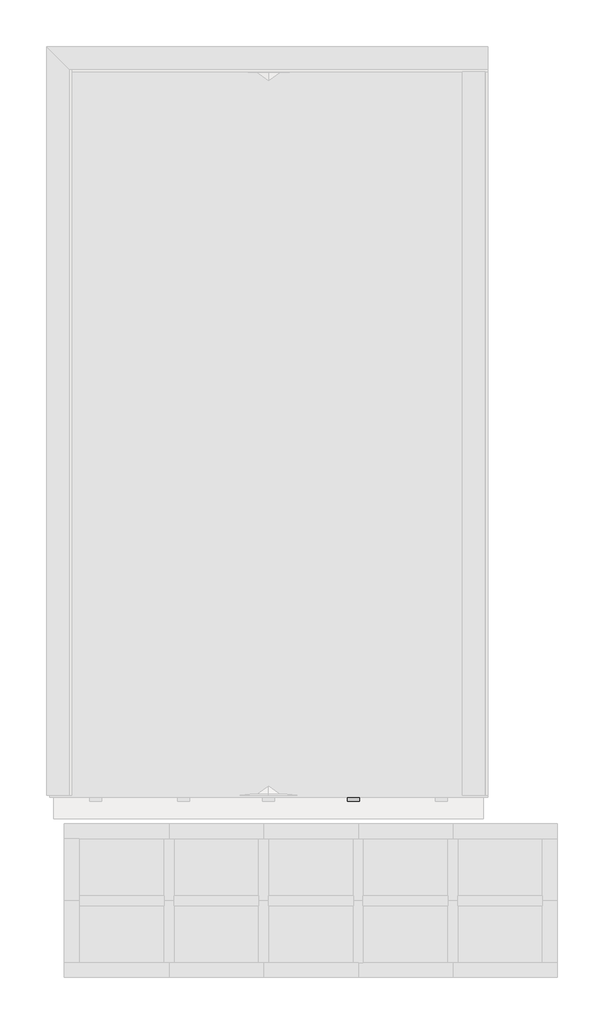
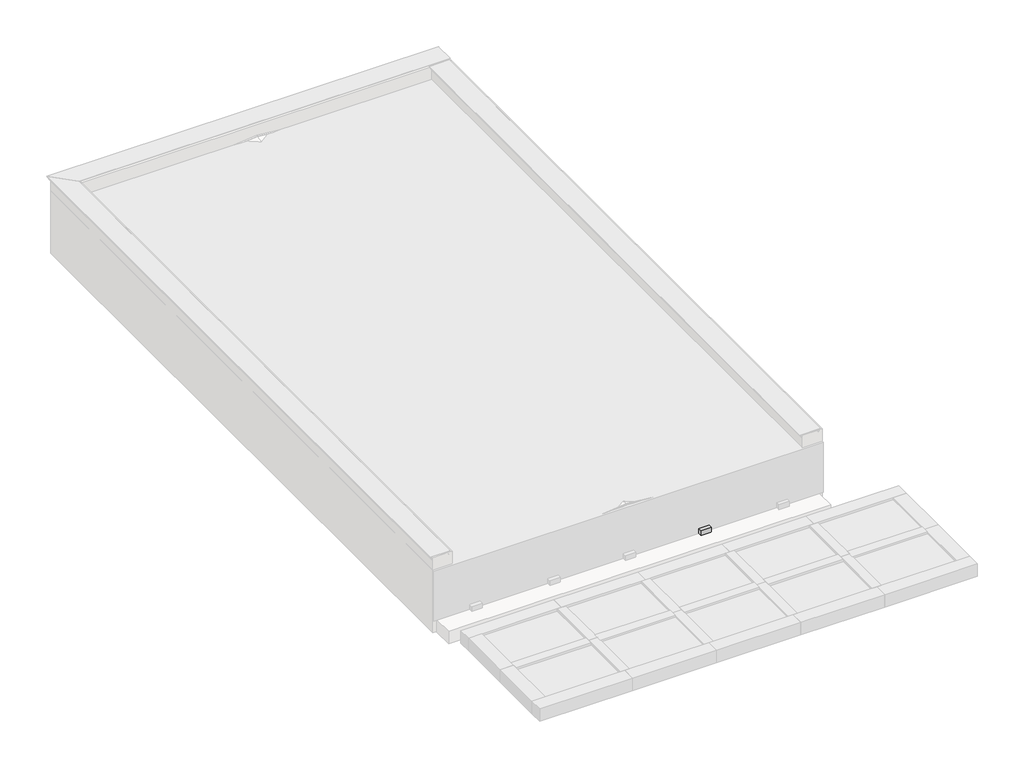
# One storey, part 2 of 3: 38 beams, 6 columns.
"""IFC4 building model written with IfcOpenShell, lengths in millimetres."""

import ifcopenshell
import ifcopenshell.guid

model = None  # the IFC model being written
_history = None  # IfcOwnerHistory: only IFC2X3 demands one
_inside = {}  # id of a spatial element -> (the spatial element, [elements in it])
_under = {}  # id of a project, library or spatial element -> (it, [spatial elements below it])
_declared = {}  # id of a project -> (the project, [libraries it declares])
_typed = {}  # id of a type object -> (the type object, [elements of that type])
_made_of = {}  # id of a material, layer set ... -> (it, [elements and type objects made of it])


def new_model(schema):
    """Start an empty IFC model of exactly this schema.

    Asked for "IFC4X3", IfcOpenShell would pick the latest addendum, in which some entities
    have other attributes; the version numbers below select the first issue.
    IFC2X3 requires an IfcOwnerHistory on every rooted entity: one is made here for all.
    """
    global model, _history
    if schema == "IFC4X3":
        model = ifcopenshell.file(schema_version=(4, 3, 0, 0))
    else:
        model = ifcopenshell.file(schema=schema)
    _inside.clear()
    _under.clear()
    _declared.clear()
    _typed.clear()
    _made_of.clear()
    _history = None
    if model.schema == "IFC2X3":
        org = make("IfcOrganization", Name="unknown")
        user = make(
            "IfcPersonAndOrganization",
            ThePerson=make("IfcPerson", FamilyName="unknown"),
            TheOrganization=org,
        )
        app = make(
            "IfcApplication",
            ApplicationDeveloper=org,
            Version="unknown",
            ApplicationFullName="unknown",
            ApplicationIdentifier="unknown",
        )
        _history = make(
            "IfcOwnerHistory",
            OwningUser=user,
            OwningApplication=app,
            ChangeAction="ADDED",
            CreationDate=0,
        )
    return model


def make(cls, **values):
    """One entity of the class cls with the attributes given. An attribute that is None is left unset."""
    return model.create_entity(
        cls, **{name: value for name, value in values.items() if value is not None}
    )


def rooted(cls, **values):
    """An entity with a GlobalId (a new one), such as an element, a storey or a relation."""
    return make(cls, GlobalId=ifcopenshell.guid.new(), OwnerHistory=_history, **values)


def si_unit(unit_type, name, prefix=None):
    """IfcSIUnit, for example si_unit("LENGTHUNIT", "METRE", prefix="MILLI")."""
    return make("IfcSIUnit", UnitType=unit_type, Prefix=prefix, Name=name)


def assignment(units):
    """IfcUnitAssignment: the units of a project."""
    return None if units is None else make("IfcUnitAssignment", Units=units)


def point(xyz):
    """IfcCartesianPoint."""
    return None if xyz is None else make("IfcCartesianPoint", Coordinates=xyz)


def direction(xyz):
    """IfcDirection."""
    return None if xyz is None else make("IfcDirection", DirectionRatios=xyz)


def frame(location, z_axis=None, x_axis=None):
    """IfcAxis2Placement3D, a coordinate frame: its origin and axes. An axis left out is left unset."""
    return make(
        "IfcAxis2Placement3D",
        Location=point(location),
        Axis=direction(z_axis),
        RefDirection=direction(x_axis),
    )


def frame_2d(location, x_axis=None):
    """IfcAxis2Placement2D, a coordinate frame in the plane: its origin and x axis."""
    return make(
        "IfcAxis2Placement2D", Location=point(location), RefDirection=direction(x_axis)
    )


def origin():
    """The frame at (0, 0, 0) with its axes left unset."""
    return frame((0.0, 0.0, 0.0))


def place(relative_to, where):
    """IfcLocalPlacement: puts the frame where relative to a parent placement (None: the world)."""
    return make(
        "IfcLocalPlacement", PlacementRelTo=relative_to, RelativePlacement=where
    )


def context(
    kind, dimensions, precision=None, world=None, true_north=None, identifier=None
):
    """IfcGeometricRepresentationContext, for example the 3D "Model" context."""
    return make(
        "IfcGeometricRepresentationContext",
        ContextIdentifier=identifier,
        ContextType=kind,
        CoordinateSpaceDimension=dimensions,
        Precision=precision,
        WorldCoordinateSystem=world,
        TrueNorth=true_north,
    )


def project(units=None, contexts=None):
    """IfcProject with its units and contexts."""
    return rooted(
        "IfcProject",
        Name="project",
        RepresentationContexts=contexts,
        UnitsInContext=assignment(units),
    )


def spatial(cls, under=None, at=None, **own):
    """A site, building, storey or space (cls), placed at a placement, below another one or the project."""
    s = rooted(cls, ObjectPlacement=at, **own)
    if under is not None:
        _under.setdefault(under.id(), (under, []))[1].append(s)
    return s


def polyline(points):
    """IfcPolyline through the points."""
    return make("IfcPolyline", Points=[point(p) for p in points])


def circle_curve(where, radius):
    """IfcCircle in the frame where."""
    return make("IfcCircle", Position=where, Radius=radius)


def trimmed(basis, trim1, trim2, sense, master):
    """IfcTrimmedCurve: the piece of a basis curve between two trims."""
    return make(
        "IfcTrimmedCurve",
        BasisCurve=basis,
        Trim1=trim1,
        Trim2=trim2,
        SenseAgreement=sense,
        MasterRepresentation=master,
    )


def segment(curve, same_sense, transition):
    """IfcCompositeCurveSegment."""
    return make(
        "IfcCompositeCurveSegment",
        Transition=transition,
        SameSense=same_sense,
        ParentCurve=curve,
    )


def composite_curve(segments, self_intersect=None):
    """IfcCompositeCurve: segments joined end to end."""
    return make("IfcCompositeCurve", Segments=segments, SelfIntersect=self_intersect)


def outline(outer, holes=None, kind="AREA"):
    """IfcArbitraryClosedProfileDef: a profile drawn as a closed curve; with holes, ...WithVoids."""
    if holes is None:
        return make("IfcArbitraryClosedProfileDef", ProfileType=kind, OuterCurve=outer)
    return make(
        "IfcArbitraryProfileDefWithVoids",
        ProfileType=kind,
        OuterCurve=outer,
        InnerCurves=holes,
    )


def extrude(swept, where, along, depth):
    """IfcExtrudedAreaSolid: the profile swept, set in the frame where, extruded along a direction by depth."""
    return make(
        "IfcExtrudedAreaSolid",
        SweptArea=swept,
        Position=where,
        ExtrudedDirection=direction(along),
        Depth=depth,
    )


def shape(context_of_items, identifier, shape_type, items):
    """IfcShapeRepresentation: the items that make up one representation, for example the "Body"."""
    return make(
        "IfcShapeRepresentation",
        ContextOfItems=context_of_items,
        RepresentationIdentifier=identifier,
        RepresentationType=shape_type,
        Items=items,
    )


def source(mapping_origin, context_of_items, identifier, shape_type, items):
    """IfcRepresentationMap: a shape defined once, which mapped items show again and again."""
    return make(
        "IfcRepresentationMap",
        MappingOrigin=mapping_origin,
        MappedRepresentation=shape(context_of_items, identifier, shape_type, items),
    )


def transform(
    local_origin,
    x_axis=None,
    y_axis=None,
    z_axis=None,
    scale=None,
    scale2=None,
    scale3=None,
    uniform=True,
):
    """IfcCartesianTransformationOperator3D, or its non-uniform kind. x_axis, y_axis, z_axis: its Axis1, 2, 3."""
    if uniform:
        return make(
            "IfcCartesianTransformationOperator3D",
            Axis1=direction(x_axis),
            Axis2=direction(y_axis),
            LocalOrigin=point(local_origin),
            Scale=scale,
            Axis3=direction(z_axis),
        )
    return make(
        "IfcCartesianTransformationOperator3DnonUniform",
        Axis1=direction(x_axis),
        Axis2=direction(y_axis),
        LocalOrigin=point(local_origin),
        Scale=scale,
        Axis3=direction(z_axis),
        Scale2=scale2,
        Scale3=scale3,
    )


def mapped(mapping_source, mapping_target):
    """IfcMappedItem: shows the shape of a source again, moved by a transform."""
    return make(
        "IfcMappedItem", MappingSource=mapping_source, MappingTarget=mapping_target
    )


def made_of(thing, what):
    """Note that an element or type object is made of a material, layer set ...; save() writes the relation."""
    if what is not None:
        _made_of.setdefault(what.id(), (what, []))[1].append(thing)
    return thing


def element(
    cls,
    number,
    at=None,
    inside=None,
    cuts=None,
    type_object=None,
    material=None,
    context=None,
    identifier="Body",
    shape_type=None,
    held_by="IfcProductDefinitionShape",
    body=None,
    shapes=None,
    **own,
):
    """One element of the class cls, such as IfcWall. Its Tag is "e" and its number.

    at: its placement. inside: the storey or other place that contains it. cuts: it is an
    opening in that element (IfcRelVoidsElement). A single representation is given by context,
    identifier, shape_type and body (its items); several are given by shapes. held_by: the class
    of the entity that holds the representations. save() writes the other relations.
    """
    e = rooted(cls, Tag="e%d" % number, ObjectPlacement=at, **own)
    if body is not None:
        shapes = [shape(context, identifier, shape_type, body)]
    if shapes is not None:
        e.Representation = make(held_by, Representations=shapes)
    if inside is not None:
        _inside.setdefault(inside.id(), (inside, []))[1].append(e)
    if cuts is not None:
        rooted(
            "IfcRelVoidsElement", RelatingBuildingElement=cuts, RelatedOpeningElement=e
        )
    if type_object is not None:
        _typed.setdefault(type_object.id(), (type_object, []))[1].append(e)
    return made_of(e, material)


def aggregate(whole, parts):
    """IfcRelAggregates: a whole, such as a stair, and the parts it consists of."""
    return rooted("IfcRelAggregates", RelatingObject=whole, RelatedObjects=parts)


def save(model, path):
    """Write the relations noted so far, then the file.

    IfcRelAggregates (storeys below a building ...), IfcRelContainedInSpatialStructure (elements
    in a storey), IfcRelDefinesByType, IfcRelAssociatesMaterial and IfcRelDeclares: one each for
    every whole, place, type object, material and project.
    """
    for whole, parts in _under.values():
        aggregate(whole, parts)
    for where, things in _inside.values():
        rooted(
            "IfcRelContainedInSpatialStructure",
            RelatedElements=things,
            RelatingStructure=where,
        )
    for kind, things in _typed.values():
        rooted("IfcRelDefinesByType", RelatedObjects=things, RelatingType=kind)
    for what, things in _made_of.values():
        rooted("IfcRelAssociatesMaterial", RelatedObjects=things, RelatingMaterial=what)
    for by, libraries in _declared.values():
        rooted("IfcRelDeclares", RelatingContext=by, RelatedDefinitions=libraries)
    model.write(path)


def cumeeira_telha_ondulada_fibrocimento_28917381(model_context):
    return source(origin(), model_context, "Body", "SweptSolid", [
        extrude(outline(composite_curve([segment(polyline([(58.3970135, 42.4437972), (53.9055884, 40.2467307)]), True, "CONTINUOUS"), segment(trimmed(circle_curve(frame_2d((-1.6029865, 13.0936483)), 61.7939461), [point((53.9055884, 40.2467307))], [point((-57.1115615, 40.2467307))], True, "CARTESIAN"), True, "CONTINUOUS"), segment(polyline([(-57.1115615, 40.2467307), (-61.6029865, 42.4437972)]), True, "CONTINUOUS"), segment(trimmed(circle_curve(frame_2d((-1.6029865, 13.0936483)), 66.7939461), [point((-61.6029865, 42.4437972))], [point((58.3970135, 42.4437972))], False, "CARTESIAN"), True, "CONTINUOUS")], self_intersect=False)), frame((-3626.5, 0.0, 0.0), z_axis=(1.0, 0.0, 0.0), x_axis=(0.0, 1.0, 0.0)), (0.0, 0.0, 1.0), 7253.0),
    ])


def viga_cumeeira_6x16cm_d80f05ee(model_context):
    return source(origin(), model_context, "Body", "SweptSolid", [
        extrude(outline(polyline([(3626.5, 30.0), (3626.5, -30.0), (-3626.5, -30.0), (-3626.5, 30.0), (3626.5, 30.0)])), frame((0.0, 0.0, -80.0), z_axis=(0.0, 0.0, 1.0), x_axis=(1.0, 0.0, 0.0)), (0.0, 0.0, 1.0), 160.0),
    ])


def column_1cffec27(model_context):
    return source(origin(), model_context, "Body", "SweptSolid", [
        extrude(outline(polyline([(30.0, 80.0), (30.0, -80.0), (-30.0, -80.0), (-30.0, 80.0), (30.0, 80.0)])), frame((0.0, 0.0, 3110.0), z_axis=(0.0, 0.0, 1.0), x_axis=(1.0, 0.0, 0.0)), (0.0, 0.0, 1.0), 238.0),
    ])


def column_35730ad5(model_context):
    return source(origin(), model_context, "Body", "SweptSolid", [
        extrude(outline(polyline([(30.0, 80.0), (30.0, -80.0), (-30.0, -80.0), (-30.0, 80.0), (30.0, 80.0)])), frame((0.0, 0.0, 3110.0), z_axis=(0.0, 0.0, 1.0), x_axis=(1.0, 0.0, 0.0)), (0.0, 0.0, 1.0), 197.9),
    ])


def column_00c463e4(model_context):
    return source(origin(), model_context, "Body", "SweptSolid", [
        extrude(outline(polyline([(30.0, 80.0), (30.0, -80.0), (-30.0, -80.0), (-30.0, 80.0), (30.0, 80.0)])), frame((0.0, 0.0, 3110.0), z_axis=(0.0, 0.0, 1.0), x_axis=(1.0, 0.0, 0.0)), (0.0, 0.0, 1.0), 109.8),
    ])


model = new_model("IFC4")

# Units and contexts
model_context = context("Model", 3, world=origin())
ifc_project = project(units=[si_unit("LENGTHUNIT", "METRE", prefix="MILLI")], contexts=[model_context])

# Site, building, storey
site = spatial("IfcSite", under=ifc_project)
building = spatial("IfcBuilding", under=site)
storey = spatial("IfcBuildingStorey", under=building, Name="COB. GARAGEM", Elevation=3050.0)

# Beams
placement = place(None, origin())
element("IfcBeam", 1, ObjectType="Madeira de lei : Berço 6x12cm", at=placement, inside=storey, context=model_context, shape_type="SweptSolid", body=[
    extrude(outline(polyline([(-9620.281307, 4423.9300153), (-9500.281307, 4423.9300153), (-9500.281307, 2423.9300153), (-9620.281307, 2423.9300153), (-9620.281307, 4423.9300153)])), frame((0.0, 0.0, 3050.0), z_axis=(0.0, 0.0, 1.0), x_axis=(1.0, 0.0, 0.0)), (0.0, 0.0, 1.0), 60.0),
])
element("IfcBeam", 2, ObjectType="Madeira de lei : Berço 6x12cm", at=placement, inside=storey, context=model_context, shape_type="SweptSolid", body=[
    extrude(outline(polyline([(-9620.281307, 2423.9300153), (-9500.281307, 2423.9300153), (-9500.281307, 423.9300153), (-9620.281307, 423.9300153), (-9620.281307, 2423.9300153)])), frame((0.0, 0.0, 3050.0), z_axis=(0.0, 0.0, 1.0), x_axis=(1.0, 0.0, 0.0)), (0.0, 0.0, 1.0), 60.0),
])
element("IfcBeam", 3, ObjectType="Madeira de lei : Berço 6x12cm", at=placement, inside=storey, context=model_context, shape_type="SweptSolid", body=[
    extrude(outline(polyline([(-8767.0824227, 4423.9300153), (-8647.0824227, 4423.9300153), (-8647.0824227, 2423.9300153), (-8767.0824227, 2423.9300153), (-8767.0824227, 4423.9300153)])), frame((0.0, 0.0, 3050.0), z_axis=(0.0, 0.0, 1.0), x_axis=(1.0, 0.0, 0.0)), (0.0, 0.0, 1.0), 60.0),
])
element("IfcBeam", 4, ObjectType="Madeira de lei : Berço 6x12cm", at=placement, inside=storey, context=model_context, shape_type="SweptSolid", body=[
    extrude(outline(polyline([(-8767.0824227, 2423.9300153), (-8647.0824227, 2423.9300153), (-8647.0824227, 423.9300153), (-8767.0824227, 423.9300153), (-8767.0824227, 2423.9300153)])), frame((0.0, 0.0, 3050.0), z_axis=(0.0, 0.0, 1.0), x_axis=(1.0, 0.0, 0.0)), (0.0, 0.0, 1.0), 60.0),
])
element("IfcBeam", 5, ObjectType="Madeira de lei : Berço 6x12cm", at=placement, inside=storey, context=model_context, shape_type="SweptSolid", body=[
    extrude(outline(polyline([(-8767.0824227, 423.9300153), (-8647.0824227, 423.9300153), (-8647.0824227, -236.0699847), (-8767.0824227, -236.0699847), (-8767.0824227, 423.9300153)])), frame((0.0, 0.0, 3050.0), z_axis=(0.0, 0.0, 1.0), x_axis=(1.0, 0.0, 0.0)), (0.0, 0.0, 1.0), 60.0),
])
element("IfcBeam", 6, ObjectType="Madeira de lei : Berço 6x12cm", at=placement, inside=storey, context=model_context, shape_type="SweptSolid", body=[
    extrude(outline(polyline([(-10473.4801913, 4423.9300153), (-10353.4801913, 4423.9300153), (-10353.4801913, 2423.9300153), (-10473.4801913, 2423.9300153), (-10473.4801913, 4423.9300153)])), frame((0.0, 0.0, 3050.0), z_axis=(0.0, 0.0, 1.0), x_axis=(1.0, 0.0, 0.0)), (0.0, 0.0, 1.0), 60.0),
])
element("IfcBeam", 7, ObjectType="Madeira de lei : Berço 6x12cm", at=placement, inside=storey, context=model_context, shape_type="SweptSolid", body=[
    extrude(outline(polyline([(-11356.5301913, 4423.9300153), (-11236.5301913, 4423.9300153), (-11236.5301913, 2423.9300153), (-11356.5301913, 2423.9300153), (-11356.5301913, 4423.9300153)])), frame((0.0, 0.0, 3050.0), z_axis=(0.0, 0.0, 1.0), x_axis=(1.0, 0.0, 0.0)), (0.0, 0.0, 1.0), 60.0),
])
cumeeira_telha_ondulada_fibrocimento_shape = cumeeira_telha_ondulada_fibrocimento_28917381(model_context)
element("IfcBeam", 8, ObjectType="Cumeeira Telha Ondulada : Fibrocimento", at=placement, inside=storey, context=model_context, shape_type="MappedRepresentation", body=[
    mapped(cumeeira_telha_ondulada_fibrocimento_shape, transform((-9560.281307, 3455.9300153, 3545.9751229), x_axis=(0.0, -1.0, 0.0), y_axis=(1.0, 0.0, 0.0), z_axis=(0.0, 0.0, 1.0))),
])
element("IfcBeam", 9, ObjectType="Telha Ondulada : Fibrocimento", at=placement, inside=storey, context=model_context, shape_type="SweptSolid", body=[
    extrude(outline(composite_curve([segment(trimmed(circle_curve(frame_2d((-58.7002979, -53.2060538)), 66.7939461), [point((-29.350149, 6.7939462))], [point((-29.350149, -113.2060538))], False, "CARTESIAN"), True, "CONTINUOUS"), segment(polyline([(-29.350149, -113.2060538), (-31.5472155, -108.7146288)]), True, "CONTINUOUS"), segment(trimmed(circle_curve(frame_2d((-58.7002979, -53.2060538)), 61.7939461), [point((-31.5472155, -108.7146288))], [point((-31.5472155, 2.3025211))], True, "CARTESIAN"), True, "CONTINUOUS"), segment(trimmed(circle_curve(frame_2d((0.0, 66.7939462)), 71.7939461), [point((-31.5472155, 2.3025211))], [point((-31.5472155, 131.2853712))], False, "CARTESIAN"), True, "CONTINUOUS"), segment(polyline([(-31.5472155, 131.2853712), (-29.350149, 126.7939462)]), True, "CONTINUOUS"), segment(trimmed(circle_curve(frame_2d((0.0, 66.7939462)), 66.7939461), [point((-29.350149, 126.7939462))], [point((-29.350149, 6.7939462))], True, "CARTESIAN"), True, "CONTINUOUS")], self_intersect=False)), frame((-11446.918865, 2229.326948, 3394.3067746), z_axis=(0.9950371902099892, 0.0, 0.09950371902099919), x_axis=(-0.09950371902099919, 0.0, 0.9950371902099892)), (0.0, 0.0, 1.0), 1886.8678854),
])
element("IfcBeam", 10, ObjectType="Telha Ondulada : Fibrocimento", at=placement, inside=storey, context=model_context, shape_type="SweptSolid", body=[
    extrude(outline(composite_curve([segment(trimmed(circle_curve(frame_2d((-58.7002979, -53.2060538)), 66.7939461), [point((-29.350149, 6.7939462))], [point((-29.350149, -113.2060538))], False, "CARTESIAN"), True, "CONTINUOUS"), segment(polyline([(-29.350149, -113.2060538), (-31.5472155, -108.7146288)]), True, "CONTINUOUS"), segment(trimmed(circle_curve(frame_2d((-58.7002979, -53.2060538)), 61.7939461), [point((-31.5472155, -108.7146288))], [point((-31.5472155, 2.3025211))], True, "CARTESIAN"), True, "CONTINUOUS"), segment(trimmed(circle_curve(frame_2d((0.0, 66.7939462)), 71.7939461), [point((-31.5472155, 2.3025211))], [point((-31.5472155, 131.2853712))], False, "CARTESIAN"), True, "CONTINUOUS"), segment(polyline([(-31.5472155, 131.2853712), (-29.350149, 126.7939462)]), True, "CONTINUOUS"), segment(trimmed(circle_curve(frame_2d((0.0, 66.7939462)), 66.7939461), [point((-29.350149, 126.7939462))], [point((-29.350149, 6.7939462))], True, "CARTESIAN"), True, "CONTINUOUS")], self_intersect=False)), frame((-11446.918865, 2473.826948, 3394.3067746), z_axis=(0.9950371902099892, 0.0, 0.09950371902099932), x_axis=(-0.09950371902099932, 0.0, 0.9950371902099892)), (0.0, 0.0, 1.0), 1886.8678854),
])
element("IfcBeam", 11, ObjectType="Telha Ondulada : Fibrocimento", at=placement, inside=storey, context=model_context, shape_type="SweptSolid", body=[
    extrude(outline(composite_curve([segment(trimmed(circle_curve(frame_2d((-58.7002979, -53.2060538)), 66.7939461), [point((-29.350149, 6.7939462))], [point((-29.350149, -113.2060538))], False, "CARTESIAN"), True, "CONTINUOUS"), segment(polyline([(-29.350149, -113.2060538), (-31.5472155, -108.7146288)]), True, "CONTINUOUS"), segment(trimmed(circle_curve(frame_2d((-58.7002979, -53.2060538)), 61.7939461), [point((-31.5472155, -108.7146288))], [point((-31.5472155, 2.3025211))], True, "CARTESIAN"), True, "CONTINUOUS"), segment(trimmed(circle_curve(frame_2d((0.0, 66.7939462)), 71.7939461), [point((-31.5472155, 2.3025211))], [point((-31.5472155, 131.2853712))], False, "CARTESIAN"), True, "CONTINUOUS"), segment(polyline([(-31.5472155, 131.2853712), (-29.350149, 126.7939462)]), True, "CONTINUOUS"), segment(trimmed(circle_curve(frame_2d((0.0, 66.7939462)), 66.7939461), [point((-29.350149, 126.7939462))], [point((-29.350149, 6.7939462))], True, "CARTESIAN"), True, "CONTINUOUS")], self_intersect=False)), frame((-11446.918865, 2718.326948, 3394.3067746), z_axis=(0.9950371902099892, 0.0, 0.09950371902099937), x_axis=(-0.09950371902099937, 0.0, 0.9950371902099892)), (0.0, 0.0, 1.0), 1886.8678854),
])
element("IfcBeam", 12, ObjectType="Telha Ondulada : Fibrocimento", at=placement, inside=storey, context=model_context, shape_type="SweptSolid", body=[
    extrude(outline(composite_curve([segment(trimmed(circle_curve(frame_2d((-58.7002979, -53.2060538)), 66.7939461), [point((-29.350149, 6.7939462))], [point((-29.350149, -113.2060538))], False, "CARTESIAN"), True, "CONTINUOUS"), segment(polyline([(-29.350149, -113.2060538), (-31.5472155, -108.7146288)]), True, "CONTINUOUS"), segment(trimmed(circle_curve(frame_2d((-58.7002979, -53.2060538)), 61.7939461), [point((-31.5472155, -108.7146288))], [point((-31.5472155, 2.3025211))], True, "CARTESIAN"), True, "CONTINUOUS"), segment(trimmed(circle_curve(frame_2d((0.0, 66.7939462)), 71.7939461), [point((-31.5472155, 2.3025211))], [point((-31.5472155, 131.2853712))], False, "CARTESIAN"), True, "CONTINUOUS"), segment(polyline([(-31.5472155, 131.2853712), (-29.350149, 126.7939462)]), True, "CONTINUOUS"), segment(trimmed(circle_curve(frame_2d((0.0, 66.7939462)), 66.7939461), [point((-29.350149, 126.7939462))], [point((-29.350149, 6.7939462))], True, "CARTESIAN"), True, "CONTINUOUS")], self_intersect=False)), frame((-11446.918865, 2962.826948, 3394.3067746), z_axis=(0.9950371902099892, 0.0, 0.09950371902099943), x_axis=(-0.09950371902099943, 0.0, 0.9950371902099892)), (0.0, 0.0, 1.0), 1886.8678854),
])
element("IfcBeam", 13, ObjectType="Telha Ondulada : Fibrocimento", at=placement, inside=storey, context=model_context, shape_type="SweptSolid", body=[
    extrude(outline(composite_curve([segment(trimmed(circle_curve(frame_2d((-58.7002979, -53.2060538)), 66.7939461), [point((-29.350149, 6.7939462))], [point((-29.350149, -113.2060538))], False, "CARTESIAN"), True, "CONTINUOUS"), segment(polyline([(-29.350149, -113.2060538), (-31.5472155, -108.7146288)]), True, "CONTINUOUS"), segment(trimmed(circle_curve(frame_2d((-58.7002979, -53.2060538)), 61.7939461), [point((-31.5472155, -108.7146288))], [point((-31.5472155, 2.3025211))], True, "CARTESIAN"), True, "CONTINUOUS"), segment(trimmed(circle_curve(frame_2d((0.0, 66.7939462)), 71.7939461), [point((-31.5472155, 2.3025211))], [point((-31.5472155, 131.2853712))], False, "CARTESIAN"), True, "CONTINUOUS"), segment(polyline([(-31.5472155, 131.2853712), (-29.350149, 126.7939462)]), True, "CONTINUOUS"), segment(trimmed(circle_curve(frame_2d((0.0, 66.7939462)), 66.7939461), [point((-29.350149, 126.7939462))], [point((-29.350149, 6.7939462))], True, "CARTESIAN"), True, "CONTINUOUS")], self_intersect=False)), frame((-11446.918865, 3207.326948, 3394.3067746), z_axis=(0.9950371902099892, 0.0, 0.09950371902099954), x_axis=(-0.09950371902099954, 0.0, 0.9950371902099892)), (0.0, 0.0, 1.0), 1886.8678854),
])
element("IfcBeam", 14, ObjectType="Telha Ondulada : Fibrocimento", at=placement, inside=storey, context=model_context, shape_type="SweptSolid", body=[
    extrude(outline(composite_curve([segment(trimmed(circle_curve(frame_2d((-58.7002979, -53.2060538)), 66.7939461), [point((-29.350149, 6.7939462))], [point((-29.350149, -113.2060538))], False, "CARTESIAN"), True, "CONTINUOUS"), segment(polyline([(-29.350149, -113.2060538), (-31.5472155, -108.7146288)]), True, "CONTINUOUS"), segment(trimmed(circle_curve(frame_2d((-58.7002979, -53.2060538)), 61.7939461), [point((-31.5472155, -108.7146288))], [point((-31.5472155, 2.3025211))], True, "CARTESIAN"), True, "CONTINUOUS"), segment(trimmed(circle_curve(frame_2d((0.0, 66.7939462)), 71.7939461), [point((-31.5472155, 2.3025211))], [point((-31.5472155, 131.2853712))], False, "CARTESIAN"), True, "CONTINUOUS"), segment(polyline([(-31.5472155, 131.2853712), (-29.350149, 126.7939462)]), True, "CONTINUOUS"), segment(trimmed(circle_curve(frame_2d((0.0, 66.7939462)), 66.7939461), [point((-29.350149, 126.7939462))], [point((-29.350149, 6.7939462))], True, "CARTESIAN"), True, "CONTINUOUS")], self_intersect=False)), frame((-11446.918865, 3451.826948, 3394.3067746), z_axis=(0.9950371902099892, 0.0, 0.09950371902099937), x_axis=(-0.09950371902099937, 0.0, 0.9950371902099892)), (0.0, 0.0, 1.0), 1886.8678854),
])
element("IfcBeam", 15, ObjectType="Telha Ondulada : Fibrocimento", at=placement, inside=storey, context=model_context, shape_type="SweptSolid", body=[
    extrude(outline(composite_curve([segment(trimmed(circle_curve(frame_2d((-58.7002979, -53.2060538)), 66.7939461), [point((-29.350149, 6.7939462))], [point((-29.350149, -113.2060538))], False, "CARTESIAN"), True, "CONTINUOUS"), segment(polyline([(-29.350149, -113.2060538), (-31.5472155, -108.7146288)]), True, "CONTINUOUS"), segment(trimmed(circle_curve(frame_2d((-58.7002979, -53.2060538)), 61.7939461), [point((-31.5472155, -108.7146288))], [point((-31.5472155, 2.3025211))], True, "CARTESIAN"), True, "CONTINUOUS"), segment(trimmed(circle_curve(frame_2d((0.0, 66.7939462)), 71.7939461), [point((-31.5472155, 2.3025211))], [point((-31.5472155, 131.2853712))], False, "CARTESIAN"), True, "CONTINUOUS"), segment(polyline([(-31.5472155, 131.2853712), (-29.350149, 126.7939462)]), True, "CONTINUOUS"), segment(trimmed(circle_curve(frame_2d((0.0, 66.7939462)), 66.7939461), [point((-29.350149, 126.7939462))], [point((-29.350149, 6.7939462))], True, "CARTESIAN"), True, "CONTINUOUS")], self_intersect=False)), frame((-11446.918865, 3696.326948, 3394.3067746), z_axis=(0.9950371902099892, 0.0, 0.09950371902099914), x_axis=(-0.09950371902099914, 0.0, 0.9950371902099892)), (0.0, 0.0, 1.0), 1886.8678854),
])
element("IfcBeam", 16, ObjectType="Telha Ondulada : Fibrocimento", at=placement, inside=storey, context=model_context, shape_type="SweptSolid", body=[
    extrude(outline(composite_curve([segment(trimmed(circle_curve(frame_2d((-58.7002979, -53.2060538)), 66.7939461), [point((-29.350149, 6.7939462))], [point((-29.350149, -113.2060538))], False, "CARTESIAN"), True, "CONTINUOUS"), segment(polyline([(-29.350149, -113.2060538), (-31.5472155, -108.7146288)]), True, "CONTINUOUS"), segment(trimmed(circle_curve(frame_2d((-58.7002979, -53.2060538)), 61.7939461), [point((-31.5472155, -108.7146288))], [point((-31.5472155, 2.3025211))], True, "CARTESIAN"), True, "CONTINUOUS"), segment(trimmed(circle_curve(frame_2d((0.0, 66.7939462)), 71.7939461), [point((-31.5472155, 2.3025211))], [point((-31.5472155, 131.2853712))], False, "CARTESIAN"), True, "CONTINUOUS"), segment(polyline([(-31.5472155, 131.2853712), (-29.350149, 126.7939462)]), True, "CONTINUOUS"), segment(trimmed(circle_curve(frame_2d((0.0, 66.7939462)), 66.7939461), [point((-29.350149, 126.7939462))], [point((-29.350149, 6.7939462))], True, "CARTESIAN"), True, "CONTINUOUS")], self_intersect=False)), frame((-11446.918865, 3940.826948, 3394.3067746), z_axis=(0.9950371902099892, 0.0, 0.09950371902099948), x_axis=(-0.09950371902099948, 0.0, 0.9950371902099892)), (0.0, 0.0, 1.0), 1886.8678854),
])
element("IfcBeam", 17, ObjectType="Telha Ondulada : Fibrocimento", at=placement, inside=storey, context=model_context, shape_type="SweptSolid", body=[
    extrude(outline(composite_curve([segment(trimmed(circle_curve(frame_2d((-58.7002979, -53.2060538)), 66.7939461), [point((-29.350149, 6.7939462))], [point((-29.350149, -113.2060538))], False, "CARTESIAN"), True, "CONTINUOUS"), segment(polyline([(-29.350149, -113.2060538), (-31.5472155, -108.7146288)]), True, "CONTINUOUS"), segment(trimmed(circle_curve(frame_2d((-58.7002979, -53.2060538)), 61.7939461), [point((-31.5472155, -108.7146288))], [point((-31.5472155, 2.3025211))], True, "CARTESIAN"), True, "CONTINUOUS"), segment(trimmed(circle_curve(frame_2d((0.0, 66.7939462)), 71.7939461), [point((-31.5472155, 2.3025211))], [point((-31.5472155, 131.2853712))], False, "CARTESIAN"), True, "CONTINUOUS"), segment(polyline([(-31.5472155, 131.2853712), (-29.350149, 126.7939462)]), True, "CONTINUOUS"), segment(trimmed(circle_curve(frame_2d((0.0, 66.7939462)), 66.7939461), [point((-29.350149, 126.7939462))], [point((-29.350149, 6.7939462))], True, "CARTESIAN"), True, "CONTINUOUS")], self_intersect=False)), frame((-11446.918865, 4185.326948, 3394.3067746), z_axis=(0.9950371902099892, 0.0, 0.09950371902099932), x_axis=(-0.09950371902099932, 0.0, 0.9950371902099892)), (0.0, 0.0, 1.0), 1886.8678854),
])
element("IfcBeam", 18, ObjectType="Telha Ondulada : Fibrocimento", at=placement, inside=storey, context=model_context, shape_type="SweptSolid", body=[
    extrude(outline(composite_curve([segment(trimmed(circle_curve(frame_2d((-58.7002979, -53.2060538)), 66.7939461), [point((-29.350149, 6.7939462))], [point((-29.350149, -113.2060538))], False, "CARTESIAN"), True, "CONTINUOUS"), segment(polyline([(-29.350149, -113.2060538), (-31.5472155, -108.7146288)]), True, "CONTINUOUS"), segment(trimmed(circle_curve(frame_2d((-58.7002979, -53.2060538)), 61.7939461), [point((-31.5472155, -108.7146288))], [point((-31.5472155, 2.3025211))], True, "CARTESIAN"), True, "CONTINUOUS"), segment(trimmed(circle_curve(frame_2d((0.0, 66.7939462)), 71.7939461), [point((-31.5472155, 2.3025211))], [point((-31.5472155, 131.2853712))], False, "CARTESIAN"), True, "CONTINUOUS"), segment(polyline([(-31.5472155, 131.2853712), (-29.350149, 126.7939462)]), True, "CONTINUOUS"), segment(trimmed(circle_curve(frame_2d((0.0, 66.7939462)), 66.7939461), [point((-29.350149, 126.7939462))], [point((-29.350149, 6.7939462))], True, "CARTESIAN"), True, "CONTINUOUS")], self_intersect=False)), frame((-11446.918865, 4429.826948, 3394.3067746), z_axis=(0.9950371902099892, 0.0, 0.09950371902099943), x_axis=(-0.09950371902099943, 0.0, 0.9950371902099892)), (0.0, 0.0, 1.0), 1886.8678854),
])
element("IfcBeam", 19, ObjectType="Telha Ondulada : Fibrocimento", at=placement, inside=storey, context=model_context, shape_type="SweptSolid", body=[
    extrude(outline(composite_curve([segment(trimmed(circle_curve(frame_2d((-58.7002979, -53.2060538)), 66.7939461), [point((-29.350149, 6.7939462))], [point((-29.350149, -113.2060538))], False, "CARTESIAN"), True, "CONTINUOUS"), segment(polyline([(-29.350149, -113.2060538), (-31.5472155, -108.7146288)]), True, "CONTINUOUS"), segment(trimmed(circle_curve(frame_2d((-58.7002979, -53.2060538)), 61.7939461), [point((-31.5472155, -108.7146288))], [point((-31.5472155, 2.3025211))], True, "CARTESIAN"), True, "CONTINUOUS"), segment(trimmed(circle_curve(frame_2d((0.0, 66.7939462)), 71.7939461), [point((-31.5472155, 2.3025211))], [point((-31.5472155, 131.2853712))], False, "CARTESIAN"), True, "CONTINUOUS"), segment(polyline([(-31.5472155, 131.2853712), (-29.350149, 126.7939462)]), True, "CONTINUOUS"), segment(trimmed(circle_curve(frame_2d((0.0, 66.7939462)), 66.7939461), [point((-29.350149, 126.7939462))], [point((-29.350149, 6.7939462))], True, "CARTESIAN"), True, "CONTINUOUS")], self_intersect=False)), frame((-11446.918865, 4674.326948, 3394.3067746), z_axis=(0.9950371902099892, 0.0, 0.09950371902099943), x_axis=(-0.09950371902099943, 0.0, 0.9950371902099892)), (0.0, 0.0, 1.0), 1886.8678854),
])
element("IfcBeam", 20, ObjectType="Telha Ondulada : Fibrocimento", at=placement, inside=storey, context=model_context, shape_type="SweptSolid", body=[
    extrude(outline(composite_curve([segment(trimmed(circle_curve(frame_2d((-58.7002979, -53.2060538)), 66.7939461), [point((-29.350149, 6.7939462))], [point((-29.350149, -113.2060538))], False, "CARTESIAN"), True, "CONTINUOUS"), segment(polyline([(-29.350149, -113.2060538), (-31.5472155, -108.7146288)]), True, "CONTINUOUS"), segment(trimmed(circle_curve(frame_2d((-58.7002979, -53.2060538)), 61.7939461), [point((-31.5472155, -108.7146288))], [point((-31.5472155, 2.3025211))], True, "CARTESIAN"), True, "CONTINUOUS"), segment(trimmed(circle_curve(frame_2d((0.0, 66.7939462)), 71.7939461), [point((-31.5472155, 2.3025211))], [point((-31.5472155, 131.2853712))], False, "CARTESIAN"), True, "CONTINUOUS"), segment(polyline([(-31.5472155, 131.2853712), (-29.350149, 126.7939462)]), True, "CONTINUOUS"), segment(trimmed(circle_curve(frame_2d((0.0, 66.7939462)), 66.7939461), [point((-29.350149, 126.7939462))], [point((-29.350149, 6.7939462))], True, "CARTESIAN"), True, "CONTINUOUS")], self_intersect=False)), frame((-11446.918865, 4918.826948, 3394.3067746), z_axis=(0.9950371902099892, 0.0, 0.09950371902099903), x_axis=(-0.09950371902099903, 0.0, 0.9950371902099892)), (0.0, 0.0, 1.0), 1886.8678854),
])
element("IfcBeam", 21, ObjectType="Telha Ondulada : Fibrocimento", at=placement, inside=storey, context=model_context, shape_type="SweptSolid", body=[
    extrude(outline(composite_curve([segment(trimmed(circle_curve(frame_2d((0.0, 66.7939462)), 66.7939461), [point((29.350149, 6.7939462))], [point((29.350149, 126.7939462))], True, "CARTESIAN"), True, "CONTINUOUS"), segment(polyline([(29.350149, 126.7939462), (31.5472155, 131.2853712)]), True, "CONTINUOUS"), segment(trimmed(circle_curve(frame_2d((0.0, 66.7939462)), 71.7939461), [point((31.5472155, 131.2853712))], [point((31.5472155, 2.3025211))], False, "CARTESIAN"), True, "CONTINUOUS"), segment(trimmed(circle_curve(frame_2d((58.7002979, -53.2060538)), 61.7939461), [point((31.5472155, 2.3025211))], [point((31.5472155, -108.7146288))], True, "CARTESIAN"), True, "CONTINUOUS"), segment(polyline([(31.5472155, -108.7146288), (29.350149, -113.2060538)]), True, "CONTINUOUS"), segment(trimmed(circle_curve(frame_2d((58.7002979, -53.2060538)), 66.7939461), [point((29.350149, -113.2060538))], [point((29.350149, 6.7939462))], False, "CARTESIAN"), True, "CONTINUOUS")], self_intersect=False)), frame((-7673.6437489, 28.826948, 3394.3067746), z_axis=(-0.9950371902099892, 0.0, 0.09950371902099979), x_axis=(-0.09950371902099979, 0.0, -0.9950371902099892)), (0.0, 0.0, 1.0), 1886.8678854),
])
element("IfcBeam", 22, ObjectType="Telha Ondulada : Fibrocimento", at=placement, inside=storey, context=model_context, shape_type="SweptSolid", body=[
    extrude(outline(composite_curve([segment(trimmed(circle_curve(frame_2d((0.0, 66.7939462)), 66.7939461), [point((29.350149, 6.7939462))], [point((29.350149, 126.7939462))], True, "CARTESIAN"), True, "CONTINUOUS"), segment(polyline([(29.350149, 126.7939462), (31.5472155, 131.2853712)]), True, "CONTINUOUS"), segment(trimmed(circle_curve(frame_2d((0.0, 66.7939462)), 71.7939461), [point((31.5472155, 131.2853712))], [point((31.5472155, 2.3025211))], False, "CARTESIAN"), True, "CONTINUOUS"), segment(trimmed(circle_curve(frame_2d((58.7002979, -53.2060538)), 61.7939461), [point((31.5472155, 2.3025211))], [point((31.5472155, -108.7146288))], True, "CARTESIAN"), True, "CONTINUOUS"), segment(polyline([(31.5472155, -108.7146288), (29.350149, -113.2060538)]), True, "CONTINUOUS"), segment(trimmed(circle_curve(frame_2d((58.7002979, -53.2060538)), 66.7939461), [point((29.350149, -113.2060538))], [point((29.350149, 6.7939462))], False, "CARTESIAN"), True, "CONTINUOUS")], self_intersect=False)), frame((-7673.6437489, 273.326948, 3394.3067746), z_axis=(-0.9950371902099892, 0.0, 0.09950371902099979), x_axis=(-0.09950371902099979, 0.0, -0.9950371902099892)), (0.0, 0.0, 1.0), 1886.8678854),
])
element("IfcBeam", 23, ObjectType="Telha Ondulada : Fibrocimento", at=placement, inside=storey, context=model_context, shape_type="SweptSolid", body=[
    extrude(outline(composite_curve([segment(trimmed(circle_curve(frame_2d((0.0, 66.7939462)), 66.7939461), [point((29.350149, 6.7939462))], [point((29.350149, 126.7939462))], True, "CARTESIAN"), True, "CONTINUOUS"), segment(polyline([(29.350149, 126.7939462), (31.5472155, 131.2853712)]), True, "CONTINUOUS"), segment(trimmed(circle_curve(frame_2d((0.0, 66.7939462)), 71.7939461), [point((31.5472155, 131.2853712))], [point((31.5472155, 2.3025211))], False, "CARTESIAN"), True, "CONTINUOUS"), segment(trimmed(circle_curve(frame_2d((58.7002979, -53.2060538)), 61.7939461), [point((31.5472155, 2.3025211))], [point((31.5472155, -108.7146288))], True, "CARTESIAN"), True, "CONTINUOUS"), segment(polyline([(31.5472155, -108.7146288), (29.350149, -113.2060538)]), True, "CONTINUOUS"), segment(trimmed(circle_curve(frame_2d((58.7002979, -53.2060538)), 66.7939461), [point((29.350149, -113.2060538))], [point((29.350149, 6.7939462))], False, "CARTESIAN"), True, "CONTINUOUS")], self_intersect=False)), frame((-7673.6437489, 517.826948, 3394.3067746), z_axis=(-0.9950371902099892, 0.0, 0.09950371902099979), x_axis=(-0.09950371902099979, 0.0, -0.9950371902099892)), (0.0, 0.0, 1.0), 1886.8678854),
])
element("IfcBeam", 24, ObjectType="Telha Ondulada : Fibrocimento", at=placement, inside=storey, context=model_context, shape_type="SweptSolid", body=[
    extrude(outline(composite_curve([segment(trimmed(circle_curve(frame_2d((0.0, 66.7939462)), 66.7939461), [point((29.350149, 6.7939462))], [point((29.350149, 126.7939462))], True, "CARTESIAN"), True, "CONTINUOUS"), segment(polyline([(29.350149, 126.7939462), (31.5472155, 131.2853712)]), True, "CONTINUOUS"), segment(trimmed(circle_curve(frame_2d((0.0, 66.7939462)), 71.7939461), [point((31.5472155, 131.2853712))], [point((31.5472155, 2.3025211))], False, "CARTESIAN"), True, "CONTINUOUS"), segment(trimmed(circle_curve(frame_2d((58.7002979, -53.2060538)), 61.7939461), [point((31.5472155, 2.3025211))], [point((31.5472155, -108.7146288))], True, "CARTESIAN"), True, "CONTINUOUS"), segment(polyline([(31.5472155, -108.7146288), (29.350149, -113.2060538)]), True, "CONTINUOUS"), segment(trimmed(circle_curve(frame_2d((58.7002979, -53.2060538)), 66.7939461), [point((29.350149, -113.2060538))], [point((29.350149, 6.7939462))], False, "CARTESIAN"), True, "CONTINUOUS")], self_intersect=False)), frame((-7673.6437489, 762.326948, 3394.3067746), z_axis=(-0.9950371902099892, 0.0, 0.09950371902099979), x_axis=(-0.09950371902099979, 0.0, -0.9950371902099892)), (0.0, 0.0, 1.0), 1886.8678854),
])
element("IfcBeam", 25, ObjectType="Telha Ondulada : Fibrocimento", at=placement, inside=storey, context=model_context, shape_type="SweptSolid", body=[
    extrude(outline(composite_curve([segment(trimmed(circle_curve(frame_2d((0.0, 66.7939462)), 66.7939461), [point((29.350149, 6.7939462))], [point((29.350149, 126.7939462))], True, "CARTESIAN"), True, "CONTINUOUS"), segment(polyline([(29.350149, 126.7939462), (31.5472155, 131.2853712)]), True, "CONTINUOUS"), segment(trimmed(circle_curve(frame_2d((0.0, 66.7939462)), 71.7939461), [point((31.5472155, 131.2853712))], [point((31.5472155, 2.3025211))], False, "CARTESIAN"), True, "CONTINUOUS"), segment(trimmed(circle_curve(frame_2d((58.7002979, -53.2060538)), 61.7939461), [point((31.5472155, 2.3025211))], [point((31.5472155, -108.7146288))], True, "CARTESIAN"), True, "CONTINUOUS"), segment(polyline([(31.5472155, -108.7146288), (29.350149, -113.2060538)]), True, "CONTINUOUS"), segment(trimmed(circle_curve(frame_2d((58.7002979, -53.2060538)), 66.7939461), [point((29.350149, -113.2060538))], [point((29.350149, 6.7939462))], False, "CARTESIAN"), True, "CONTINUOUS")], self_intersect=False)), frame((-7673.6437489, 1006.826948, 3394.3067746), z_axis=(-0.9950371902099892, 0.0, 0.09950371902099979), x_axis=(-0.09950371902099979, 0.0, -0.9950371902099892)), (0.0, 0.0, 1.0), 1886.8678854),
])
element("IfcBeam", 26, ObjectType="Telha Ondulada : Fibrocimento", at=placement, inside=storey, context=model_context, shape_type="SweptSolid", body=[
    extrude(outline(composite_curve([segment(trimmed(circle_curve(frame_2d((0.0, 66.7939462)), 66.7939461), [point((29.350149, 6.7939462))], [point((29.350149, 126.7939462))], True, "CARTESIAN"), True, "CONTINUOUS"), segment(polyline([(29.350149, 126.7939462), (31.5472155, 131.2853712)]), True, "CONTINUOUS"), segment(trimmed(circle_curve(frame_2d((0.0, 66.7939462)), 71.7939461), [point((31.5472155, 131.2853712))], [point((31.5472155, 2.3025211))], False, "CARTESIAN"), True, "CONTINUOUS"), segment(trimmed(circle_curve(frame_2d((58.7002979, -53.2060538)), 61.7939461), [point((31.5472155, 2.3025211))], [point((31.5472155, -108.7146288))], True, "CARTESIAN"), True, "CONTINUOUS"), segment(polyline([(31.5472155, -108.7146288), (29.350149, -113.2060538)]), True, "CONTINUOUS"), segment(trimmed(circle_curve(frame_2d((58.7002979, -53.2060538)), 66.7939461), [point((29.350149, -113.2060538))], [point((29.350149, 6.7939462))], False, "CARTESIAN"), True, "CONTINUOUS")], self_intersect=False)), frame((-7673.6437489, 1251.326948, 3394.3067746), z_axis=(-0.9950371902099892, 0.0, 0.09950371902099979), x_axis=(-0.09950371902099979, 0.0, -0.9950371902099892)), (0.0, 0.0, 1.0), 1886.8678854),
])
element("IfcBeam", 27, ObjectType="Telha Ondulada : Fibrocimento", at=placement, inside=storey, context=model_context, shape_type="SweptSolid", body=[
    extrude(outline(composite_curve([segment(trimmed(circle_curve(frame_2d((0.0, 66.7939462)), 66.7939461), [point((29.350149, 6.7939462))], [point((29.350149, 126.7939462))], True, "CARTESIAN"), True, "CONTINUOUS"), segment(polyline([(29.350149, 126.7939462), (31.5472155, 131.2853712)]), True, "CONTINUOUS"), segment(trimmed(circle_curve(frame_2d((0.0, 66.7939462)), 71.7939461), [point((31.5472155, 131.2853712))], [point((31.5472155, 2.3025211))], False, "CARTESIAN"), True, "CONTINUOUS"), segment(trimmed(circle_curve(frame_2d((58.7002979, -53.2060538)), 61.7939461), [point((31.5472155, 2.3025211))], [point((31.5472155, -108.7146288))], True, "CARTESIAN"), True, "CONTINUOUS"), segment(polyline([(31.5472155, -108.7146288), (29.350149, -113.2060538)]), True, "CONTINUOUS"), segment(trimmed(circle_curve(frame_2d((58.7002979, -53.2060538)), 66.7939461), [point((29.350149, -113.2060538))], [point((29.350149, 6.7939462))], False, "CARTESIAN"), True, "CONTINUOUS")], self_intersect=False)), frame((-7673.6437489, 1495.826948, 3394.3067746), z_axis=(-0.9950371902099892, 0.0, 0.09950371902099979), x_axis=(-0.09950371902099979, 0.0, -0.9950371902099892)), (0.0, 0.0, 1.0), 1886.8678854),
])
element("IfcBeam", 28, ObjectType="Telha Ondulada : Fibrocimento", at=placement, inside=storey, context=model_context, shape_type="SweptSolid", body=[
    extrude(outline(composite_curve([segment(trimmed(circle_curve(frame_2d((0.0, 66.7939462)), 66.7939461), [point((29.350149, 6.7939462))], [point((29.350149, 126.7939462))], True, "CARTESIAN"), True, "CONTINUOUS"), segment(polyline([(29.350149, 126.7939462), (31.5472155, 131.2853712)]), True, "CONTINUOUS"), segment(trimmed(circle_curve(frame_2d((0.0, 66.7939462)), 71.7939461), [point((31.5472155, 131.2853712))], [point((31.5472155, 2.3025211))], False, "CARTESIAN"), True, "CONTINUOUS"), segment(trimmed(circle_curve(frame_2d((58.7002979, -53.2060538)), 61.7939461), [point((31.5472155, 2.3025211))], [point((31.5472155, -108.7146288))], True, "CARTESIAN"), True, "CONTINUOUS"), segment(polyline([(31.5472155, -108.7146288), (29.350149, -113.2060538)]), True, "CONTINUOUS"), segment(trimmed(circle_curve(frame_2d((58.7002979, -53.2060538)), 66.7939461), [point((29.350149, -113.2060538))], [point((29.350149, 6.7939462))], False, "CARTESIAN"), True, "CONTINUOUS")], self_intersect=False)), frame((-7673.6437489, 1740.326948, 3394.3067746), z_axis=(-0.9950371902099892, 0.0, 0.09950371902099979), x_axis=(-0.09950371902099979, 0.0, -0.9950371902099892)), (0.0, 0.0, 1.0), 1886.8678854),
])
element("IfcBeam", 29, ObjectType="Telha Ondulada : Fibrocimento", at=placement, inside=storey, context=model_context, shape_type="SweptSolid", body=[
    extrude(outline(composite_curve([segment(trimmed(circle_curve(frame_2d((0.0, 66.7939462)), 66.7939461), [point((29.350149, 6.7939462))], [point((29.350149, 126.7939462))], True, "CARTESIAN"), True, "CONTINUOUS"), segment(polyline([(29.350149, 126.7939462), (31.5472155, 131.2853712)]), True, "CONTINUOUS"), segment(trimmed(circle_curve(frame_2d((0.0, 66.7939462)), 71.7939461), [point((31.5472155, 131.2853712))], [point((31.5472155, 2.3025211))], False, "CARTESIAN"), True, "CONTINUOUS"), segment(trimmed(circle_curve(frame_2d((58.7002979, -53.2060538)), 61.7939461), [point((31.5472155, 2.3025211))], [point((31.5472155, -108.7146288))], True, "CARTESIAN"), True, "CONTINUOUS"), segment(polyline([(31.5472155, -108.7146288), (29.350149, -113.2060538)]), True, "CONTINUOUS"), segment(trimmed(circle_curve(frame_2d((58.7002979, -53.2060538)), 66.7939461), [point((29.350149, -113.2060538))], [point((29.350149, 6.7939462))], False, "CARTESIAN"), True, "CONTINUOUS")], self_intersect=False)), frame((-7673.6437489, 1984.826948, 3394.3067746), z_axis=(-0.9950371902099892, 0.0, 0.09950371902099979), x_axis=(-0.09950371902099979, 0.0, -0.9950371902099892)), (0.0, 0.0, 1.0), 1886.8678854),
])
element("IfcBeam", 30, ObjectType="Telha Ondulada : Fibrocimento", at=placement, inside=storey, context=model_context, shape_type="SweptSolid", body=[
    extrude(outline(composite_curve([segment(trimmed(circle_curve(frame_2d((0.0, 66.7939462)), 66.7939461), [point((29.350149, 6.7939462))], [point((29.350149, 126.7939462))], True, "CARTESIAN"), True, "CONTINUOUS"), segment(polyline([(29.350149, 126.7939462), (31.5472155, 131.2853712)]), True, "CONTINUOUS"), segment(trimmed(circle_curve(frame_2d((0.0, 66.7939462)), 71.7939461), [point((31.5472155, 131.2853712))], [point((31.5472155, 2.3025211))], False, "CARTESIAN"), True, "CONTINUOUS"), segment(trimmed(circle_curve(frame_2d((58.7002979, -53.2060538)), 61.7939461), [point((31.5472155, 2.3025211))], [point((31.5472155, -108.7146288))], True, "CARTESIAN"), True, "CONTINUOUS"), segment(polyline([(31.5472155, -108.7146288), (29.350149, -113.2060538)]), True, "CONTINUOUS"), segment(trimmed(circle_curve(frame_2d((58.7002979, -53.2060538)), 66.7939461), [point((29.350149, -113.2060538))], [point((29.350149, 6.7939462))], False, "CARTESIAN"), True, "CONTINUOUS")], self_intersect=False)), frame((-7673.6437489, 2229.326948, 3394.3067746), z_axis=(-0.9950371902099892, 0.0, 0.09950371902099979), x_axis=(-0.09950371902099979, 0.0, -0.9950371902099892)), (0.0, 0.0, 1.0), 1886.8678854),
])
element("IfcBeam", 31, ObjectType="Telha Ondulada : Fibrocimento", at=placement, inside=storey, context=model_context, shape_type="SweptSolid", body=[
    extrude(outline(composite_curve([segment(trimmed(circle_curve(frame_2d((0.0, 66.7939462)), 66.7939461), [point((29.350149, 6.7939462))], [point((29.350149, 126.7939462))], True, "CARTESIAN"), True, "CONTINUOUS"), segment(polyline([(29.350149, 126.7939462), (31.5472155, 131.2853712)]), True, "CONTINUOUS"), segment(trimmed(circle_curve(frame_2d((0.0, 66.7939462)), 71.7939461), [point((31.5472155, 131.2853712))], [point((31.5472155, 2.3025211))], False, "CARTESIAN"), True, "CONTINUOUS"), segment(trimmed(circle_curve(frame_2d((58.7002979, -53.2060538)), 61.7939461), [point((31.5472155, 2.3025211))], [point((31.5472155, -108.7146288))], True, "CARTESIAN"), True, "CONTINUOUS"), segment(polyline([(31.5472155, -108.7146288), (29.350149, -113.2060538)]), True, "CONTINUOUS"), segment(trimmed(circle_curve(frame_2d((58.7002979, -53.2060538)), 66.7939461), [point((29.350149, -113.2060538))], [point((29.350149, 6.7939462))], False, "CARTESIAN"), True, "CONTINUOUS")], self_intersect=False)), frame((-7673.6437489, 2473.826948, 3394.3067746), z_axis=(-0.9950371902099892, 0.0, 0.09950371902099979), x_axis=(-0.09950371902099979, 0.0, -0.9950371902099892)), (0.0, 0.0, 1.0), 1886.8678854),
])
element("IfcBeam", 32, ObjectType="Telha Ondulada : Fibrocimento", at=placement, inside=storey, context=model_context, shape_type="SweptSolid", body=[
    extrude(outline(composite_curve([segment(trimmed(circle_curve(frame_2d((0.0, 66.7939462)), 66.7939461), [point((29.350149, 6.7939462))], [point((29.350149, 126.7939462))], True, "CARTESIAN"), True, "CONTINUOUS"), segment(polyline([(29.350149, 126.7939462), (31.5472155, 131.2853712)]), True, "CONTINUOUS"), segment(trimmed(circle_curve(frame_2d((0.0, 66.7939462)), 71.7939461), [point((31.5472155, 131.2853712))], [point((31.5472155, 2.3025211))], False, "CARTESIAN"), True, "CONTINUOUS"), segment(trimmed(circle_curve(frame_2d((58.7002979, -53.2060538)), 61.7939461), [point((31.5472155, 2.3025211))], [point((31.5472155, -108.7146288))], True, "CARTESIAN"), True, "CONTINUOUS"), segment(polyline([(31.5472155, -108.7146288), (29.350149, -113.2060538)]), True, "CONTINUOUS"), segment(trimmed(circle_curve(frame_2d((58.7002979, -53.2060538)), 66.7939461), [point((29.350149, -113.2060538))], [point((29.350149, 6.7939462))], False, "CARTESIAN"), True, "CONTINUOUS")], self_intersect=False)), frame((-7673.6437489, 2718.326948, 3394.3067746), z_axis=(-0.9950371902099892, 0.0, 0.09950371902099979), x_axis=(-0.09950371902099979, 0.0, -0.9950371902099892)), (0.0, 0.0, 1.0), 1886.8678854),
])
element("IfcBeam", 33, ObjectType="Telha Ondulada : Fibrocimento", at=placement, inside=storey, context=model_context, shape_type="SweptSolid", body=[
    extrude(outline(composite_curve([segment(trimmed(circle_curve(frame_2d((0.0, 66.7939462)), 66.7939461), [point((29.350149, 6.7939462))], [point((29.350149, 126.7939462))], True, "CARTESIAN"), True, "CONTINUOUS"), segment(polyline([(29.350149, 126.7939462), (31.5472155, 131.2853712)]), True, "CONTINUOUS"), segment(trimmed(circle_curve(frame_2d((0.0, 66.7939462)), 71.7939461), [point((31.5472155, 131.2853712))], [point((31.5472155, 2.3025211))], False, "CARTESIAN"), True, "CONTINUOUS"), segment(trimmed(circle_curve(frame_2d((58.7002979, -53.2060538)), 61.7939461), [point((31.5472155, 2.3025211))], [point((31.5472155, -108.7146288))], True, "CARTESIAN"), True, "CONTINUOUS"), segment(polyline([(31.5472155, -108.7146288), (29.350149, -113.2060538)]), True, "CONTINUOUS"), segment(trimmed(circle_curve(frame_2d((58.7002979, -53.2060538)), 66.7939461), [point((29.350149, -113.2060538))], [point((29.350149, 6.7939462))], False, "CARTESIAN"), True, "CONTINUOUS")], self_intersect=False)), frame((-7673.6437489, 2962.826948, 3394.3067746), z_axis=(-0.9950371902099892, 0.0, 0.09950371902099979), x_axis=(-0.09950371902099979, 0.0, -0.9950371902099892)), (0.0, 0.0, 1.0), 1886.8678854),
])
element("IfcBeam", 34, ObjectType="Telha Ondulada : Fibrocimento", at=placement, inside=storey, context=model_context, shape_type="SweptSolid", body=[
    extrude(outline(composite_curve([segment(trimmed(circle_curve(frame_2d((0.0, 66.7939462)), 66.7939461), [point((29.350149, 6.7939462))], [point((29.350149, 126.7939462))], True, "CARTESIAN"), True, "CONTINUOUS"), segment(polyline([(29.350149, 126.7939462), (31.5472155, 131.2853712)]), True, "CONTINUOUS"), segment(trimmed(circle_curve(frame_2d((0.0, 66.7939462)), 71.7939461), [point((31.5472155, 131.2853712))], [point((31.5472155, 2.3025211))], False, "CARTESIAN"), True, "CONTINUOUS"), segment(trimmed(circle_curve(frame_2d((58.7002979, -53.2060538)), 61.7939461), [point((31.5472155, 2.3025211))], [point((31.5472155, -108.7146288))], True, "CARTESIAN"), True, "CONTINUOUS"), segment(polyline([(31.5472155, -108.7146288), (29.350149, -113.2060538)]), True, "CONTINUOUS"), segment(trimmed(circle_curve(frame_2d((58.7002979, -53.2060538)), 66.7939461), [point((29.350149, -113.2060538))], [point((29.350149, 6.7939462))], False, "CARTESIAN"), True, "CONTINUOUS")], self_intersect=False)), frame((-7673.6437489, 3207.326948, 3394.3067746), z_axis=(-0.9950371902099892, 0.0, 0.09950371902099979), x_axis=(-0.09950371902099979, 0.0, -0.9950371902099892)), (0.0, 0.0, 1.0), 1886.8678854),
])
element("IfcBeam", 35, ObjectType="Telha Ondulada : Fibrocimento", at=placement, inside=storey, context=model_context, shape_type="SweptSolid", body=[
    extrude(outline(composite_curve([segment(trimmed(circle_curve(frame_2d((0.0, 66.7939462)), 66.7939461), [point((29.350149, 6.7939462))], [point((29.350149, 126.7939462))], True, "CARTESIAN"), True, "CONTINUOUS"), segment(polyline([(29.350149, 126.7939462), (31.5472155, 131.2853712)]), True, "CONTINUOUS"), segment(trimmed(circle_curve(frame_2d((0.0, 66.7939462)), 71.7939461), [point((31.5472155, 131.2853712))], [point((31.5472155, 2.3025211))], False, "CARTESIAN"), True, "CONTINUOUS"), segment(trimmed(circle_curve(frame_2d((58.7002979, -53.2060538)), 61.7939461), [point((31.5472155, 2.3025211))], [point((31.5472155, -108.7146288))], True, "CARTESIAN"), True, "CONTINUOUS"), segment(polyline([(31.5472155, -108.7146288), (29.350149, -113.2060538)]), True, "CONTINUOUS"), segment(trimmed(circle_curve(frame_2d((58.7002979, -53.2060538)), 66.7939461), [point((29.350149, -113.2060538))], [point((29.350149, 6.7939462))], False, "CARTESIAN"), True, "CONTINUOUS")], self_intersect=False)), frame((-7673.6437489, 3451.826948, 3394.3067746), z_axis=(-0.9950371902099892, 0.0, 0.09950371902099979), x_axis=(-0.09950371902099979, 0.0, -0.9950371902099892)), (0.0, 0.0, 1.0), 1886.8678854),
])
element("IfcBeam", 36, ObjectType="Telha Ondulada : Fibrocimento", at=placement, inside=storey, context=model_context, shape_type="SweptSolid", body=[
    extrude(outline(composite_curve([segment(trimmed(circle_curve(frame_2d((0.0, 66.7939462)), 66.7939461), [point((29.350149, 6.7939462))], [point((29.350149, 126.7939462))], True, "CARTESIAN"), True, "CONTINUOUS"), segment(polyline([(29.350149, 126.7939462), (31.5472155, 131.2853712)]), True, "CONTINUOUS"), segment(trimmed(circle_curve(frame_2d((0.0, 66.7939462)), 71.7939461), [point((31.5472155, 131.2853712))], [point((31.5472155, 2.3025211))], False, "CARTESIAN"), True, "CONTINUOUS"), segment(trimmed(circle_curve(frame_2d((58.7002979, -53.2060538)), 61.7939461), [point((31.5472155, 2.3025211))], [point((31.5472155, -108.7146288))], True, "CARTESIAN"), True, "CONTINUOUS"), segment(polyline([(31.5472155, -108.7146288), (29.350149, -113.2060538)]), True, "CONTINUOUS"), segment(trimmed(circle_curve(frame_2d((58.7002979, -53.2060538)), 66.7939461), [point((29.350149, -113.2060538))], [point((29.350149, 6.7939462))], False, "CARTESIAN"), True, "CONTINUOUS")], self_intersect=False)), frame((-7673.6437489, 3696.326948, 3394.3067746), z_axis=(-0.9950371902099892, 0.0, 0.09950371902099979), x_axis=(-0.09950371902099979, 0.0, -0.9950371902099892)), (0.0, 0.0, 1.0), 1886.8678854),
])
element("IfcBeam", 37, ObjectType="Telha Ondulada : Fibrocimento", at=placement, inside=storey, context=model_context, shape_type="SweptSolid", body=[
    extrude(outline(composite_curve([segment(trimmed(circle_curve(frame_2d((0.0, 66.7939462)), 66.7939461), [point((29.350149, 6.7939462))], [point((29.350149, 126.7939462))], True, "CARTESIAN"), True, "CONTINUOUS"), segment(polyline([(29.350149, 126.7939462), (31.5472155, 131.2853712)]), True, "CONTINUOUS"), segment(trimmed(circle_curve(frame_2d((0.0, 66.7939462)), 71.7939461), [point((31.5472155, 131.2853712))], [point((31.5472155, 2.3025211))], False, "CARTESIAN"), True, "CONTINUOUS"), segment(trimmed(circle_curve(frame_2d((58.7002979, -53.2060538)), 61.7939461), [point((31.5472155, 2.3025211))], [point((31.5472155, -108.7146288))], True, "CARTESIAN"), True, "CONTINUOUS"), segment(polyline([(31.5472155, -108.7146288), (29.350149, -113.2060538)]), True, "CONTINUOUS"), segment(trimmed(circle_curve(frame_2d((58.7002979, -53.2060538)), 66.7939461), [point((29.350149, -113.2060538))], [point((29.350149, 6.7939462))], False, "CARTESIAN"), True, "CONTINUOUS")], self_intersect=False)), frame((-7673.6437489, 3940.826948, 3394.3067746), z_axis=(-0.9950371902099892, 0.0, 0.09950371902099979), x_axis=(-0.09950371902099979, 0.0, -0.9950371902099892)), (0.0, 0.0, 1.0), 1886.8678854),
])
viga_cumeeira_6x16cm_shape = viga_cumeeira_6x16cm_d80f05ee(model_context)
element("IfcBeam", 38, ObjectType="Madeira de lei : Viga Cumeeira 6x16cm", at=placement, inside=storey, context=model_context, shape_type="MappedRepresentation", body=[
    mapped(viga_cumeeira_6x16cm_shape, transform((-9560.281307, 3455.9300153, 3427.8), x_axis=(0.0, -1.0, 0.0), y_axis=(1.0, 0.0, 0.0), z_axis=(0.0, 0.0, 1.0))),
])

# Columns
column_shape = column_1cffec27(model_context)
element("IfcColumn", 39, ObjectType="Madeira de lei-Coluna : Pontalete 6X16cm", at=placement, inside=storey, context=model_context, shape_type="MappedRepresentation", body=[
    mapped(column_shape, transform((-9560.281307, 3423.9300153, 0.0), x_axis=(1.0, 0.0, 0.0), y_axis=(0.0, 1.0, 0.0), z_axis=(0.0, 0.0, 1.0))),
])
element("IfcColumn", 40, ObjectType="Madeira de lei-Coluna : Pontalete 6X16cm", at=placement, inside=storey, context=model_context, shape_type="MappedRepresentation", body=[
    mapped(column_shape, transform((-9560.281307, 1423.9300153, 0.0), x_axis=(1.0, 0.0, 0.0), y_axis=(0.0, 1.0, 0.0), z_axis=(0.0, 0.0, 1.0))),
])
column_2_shape = column_35730ad5(model_context)
element("IfcColumn", 41, ObjectType="Madeira de lei-Coluna : Pontalete 6X16cm", at=placement, inside=storey, context=model_context, shape_type="MappedRepresentation", body=[
    mapped(column_2_shape, transform((-8707.0824227, 3423.9300153, 0.0), x_axis=(1.0, 0.0, 0.0), y_axis=(0.0, 1.0, 0.0), z_axis=(0.0, 0.0, 1.0))),
])
element("IfcColumn", 42, ObjectType="Madeira de lei-Coluna : Pontalete 6X16cm", at=placement, inside=storey, context=model_context, shape_type="MappedRepresentation", body=[
    mapped(column_2_shape, transform((-8707.0824227, 1423.9300153, 0.0), x_axis=(1.0, 0.0, 0.0), y_axis=(0.0, 1.0, 0.0), z_axis=(0.0, 0.0, 1.0))),
])
element("IfcColumn", 43, ObjectType="Madeira de lei-Coluna : Pontalete 6X16cm", at=placement, inside=storey, context=model_context, shape_type="MappedRepresentation", body=[
    mapped(column_2_shape, transform((-10413.4801913, 3423.9300153, 0.0), x_axis=(1.0, 0.0, 0.0), y_axis=(0.0, 1.0, 0.0), z_axis=(0.0, 0.0, 1.0))),
])
column_3_shape = column_00c463e4(model_context)
element("IfcColumn", 44, ObjectType="Madeira de lei-Coluna : Pontalete 6X16cm", at=placement, inside=storey, context=model_context, shape_type="MappedRepresentation", body=[
    mapped(column_3_shape, transform((-11296.5301913, 3423.9300153, 0.0), x_axis=(1.0, 0.0, 0.0), y_axis=(0.0, 1.0, 0.0), z_axis=(0.0, 0.0, 1.0))),
])

save(model, "model.ifc")

# Revit data of these elements
# Project information
#   Design Option = "Main Model"
#   Project Status = "Status do projeto"
#   Client Name = "JOÃO MATIAS SOARES"
#   Project Address = "RUA SÉRGIO DIAS, LOTE 30, QUADRA G, MONTE MINEIRO/MG"
#   Project Name = "CONSTRUÇÃO RESIDENCIA UNIFAMILIAR"
#   Project Number = "034/2017"
#   Zona = "ZER - 01"
#   CA Mín = "0.2"
#   CA Básico = "1"
#   CA Máx = "2"
#   TO Máx = "50"
#   Gabarito Máx = "10"
#   TP Mín = "15"
#   Área Total do Terreno = "620.00 m²"
#   Multifamiliar - Vagas Veículos/Pavto = "0"
#   Multifamiliar - Vagas Bicicletas/Pavto = "0"
#   Multifamiliar - % Vagas PNMR = "0"
#   Multifamiliar - % Vagas Motos = "0"
#   Outros - Área p/ 1 Veículo = "0.00 m²"
#   Outros - Área p/ 1 Bicicleta = "0.00 m²"
#   Outros - Área p/ 1 Utilitário = "0.00 m²"
#   Outros - % Vagas PNMR = "0"
#   Outros - % Vagas Motos = "0"
